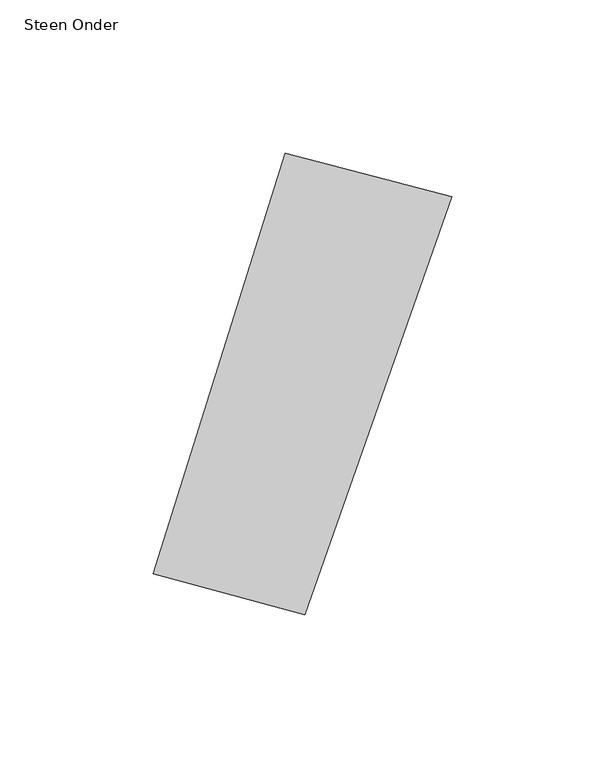
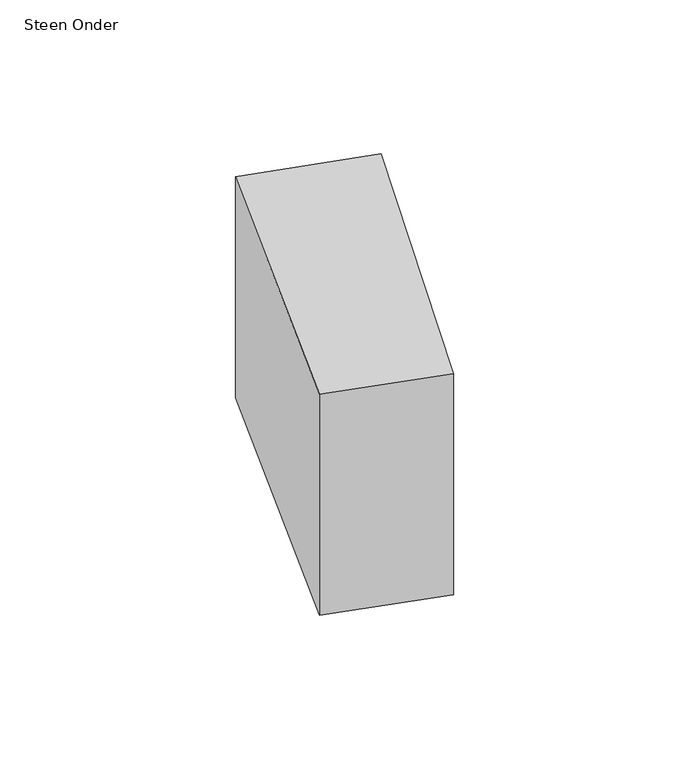
"""IFC4 building model written with IfcOpenShell, lengths in millimetres: proxy geometry, 00_GMA_steen_versie_4 : Steen Onder."""

from ifc_helpers import new_model, si_unit, origin, origin_with_axes, place, context, project, spatial, polyline, outline, extrude, source, transform, mapped, element, save


def steen_onder_a46a82f3(model_context):
    return source(origin(), model_context, "Body", "SweptSolid", [
        extrude(outline(polyline([(123.8291085, 135.8035318), (75.9854898, -0.6629545), (26.4804173, 12.7640432), (69.5946455, 149.930591), (123.8291085, 135.8035318)])), origin_with_axes(), (0.0, 0.0, 1.0), 100.0),
    ])


if __name__ == "__main__":
    model = new_model("IFC4")
    model_context = context("Model", 3, world=origin())
    ifc_project = project(units=[si_unit("LENGTHUNIT", "METRE", prefix="MILLI")], contexts=[model_context])
    site = spatial("IfcSite", under=ifc_project)
    building = spatial("IfcBuilding", under=site)
    placement = place(None, origin())
    steen_onder_shape = steen_onder_a46a82f3(model_context)
    element("IfcBuildingElementProxy", 1, Name="00_GMA_steen_versie_4 : Steen Onder", ObjectType="00_GMA_steen_versie_4 : Steen Onder", at=placement, inside=building, context=model_context, shape_type="MappedRepresentation", body=[
        mapped(steen_onder_shape, transform((0.0, 0.0, 0.0), x_axis=(1.0, 0.0, 0.0), y_axis=(0.0, 1.0, 0.0), z_axis=(0.0, 0.0, 1.0))),
    ])
    save(model, "model.ifc")

# Revit data of these elements
# Type "00_GMA_steen_versie_4 : Steen Onder"
#   StootVoegHalfBoven [instance default] = 5 mm
#   StootVoegHalf [instance default] = 5 mm
#   StootVoegBreedteOnder = 10 mm
#   StootVoegBreedteBoven = 10 mm
#   Steendikte = 100 mm
#   LintVoegOnderHalf = 0 mm
#   LintVoegOnder = 0 mm
#   LintVoegBovenHalf = 5 mm
#   LintVoegBoven = 10 mm
#   materiaal = none
#   MateriaalVoeg = none
#   Default Elevation = 0
